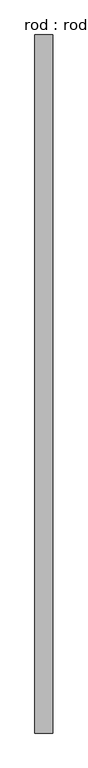
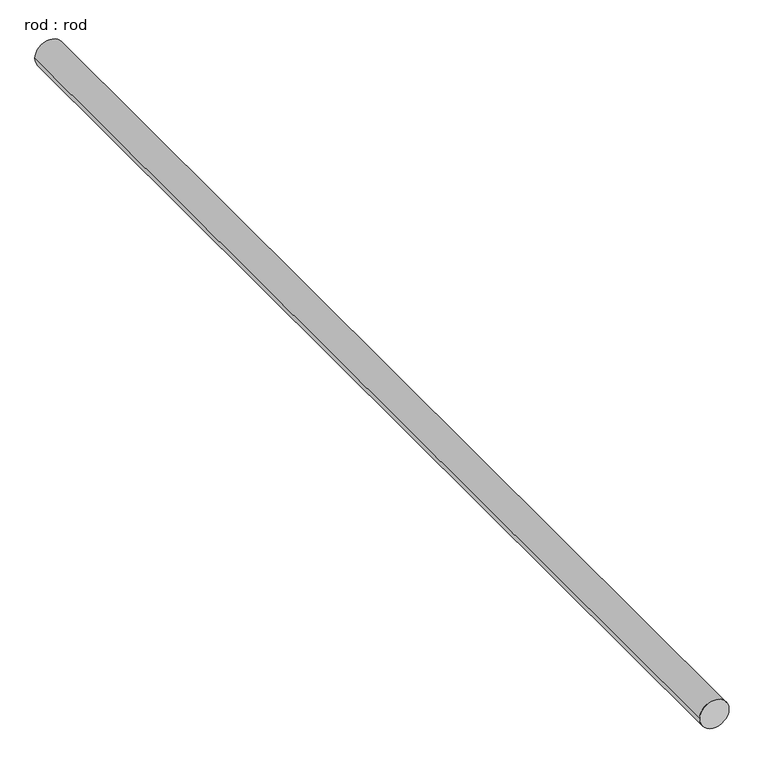
"""IFC4 building model written with IfcOpenShell, lengths in millimetres: proxy geometry, rod : rod."""

from ifc_helpers import new_model, si_unit, point, frame, frame_2d, origin, place, context, project, spatial, circle_curve, trimmed, segment, composite_curve, outline, extrude, source, transform, mapped, element, save


def rod_rod_feb64795(model_context):
    return source(origin(), model_context, "Body", "SweptSolid", [
        extrude(outline(composite_curve([segment(trimmed(circle_curve(frame_2d((0.0108462, 0.0)), 200.0), [point((0.0108462, 200.0))], [point((0.0108462, -200.0))], False, "CARTESIAN"), True, "CONTINUOUS"), segment(trimmed(circle_curve(frame_2d((0.0108462, 0.0)), 200.0), [point((0.0108462, -200.0))], [point((0.0108462, 200.0))], False, "CARTESIAN"), True, "CONTINUOUS")], self_intersect=False)), frame((0.0, -3774.342393, 0.0), z_axis=(0.0, 1.0, 0.0), x_axis=(0.0, 0.0, 1.0)), (0.0, 0.0, 1.0), 15734.1420166),
    ])


if __name__ == "__main__":
    model = new_model("IFC4")
    model_context = context("Model", 3, world=origin())
    ifc_project = project(units=[si_unit("LENGTHUNIT", "METRE", prefix="MILLI")], contexts=[model_context])
    site = spatial("IfcSite", under=ifc_project)
    building = spatial("IfcBuilding", under=site)
    placement = place(None, origin())
    rod_rod_shape = rod_rod_feb64795(model_context)
    element("IfcBuildingElementProxy", 1, Name="rod : rod", ObjectType="rod : rod", at=placement, inside=building, context=model_context, shape_type="MappedRepresentation", body=[
        mapped(rod_rod_shape, transform((0.0, 0.0, 0.0), x_axis=(1.0, 0.0, 0.0), y_axis=(0.0, 1.0, 0.0), z_axis=(0.0, 0.0, 1.0))),
    ])
    save(model, "model.ifc")

# Revit data of these elements
# Type "rod : rod"
#   Default Elevation = 0
